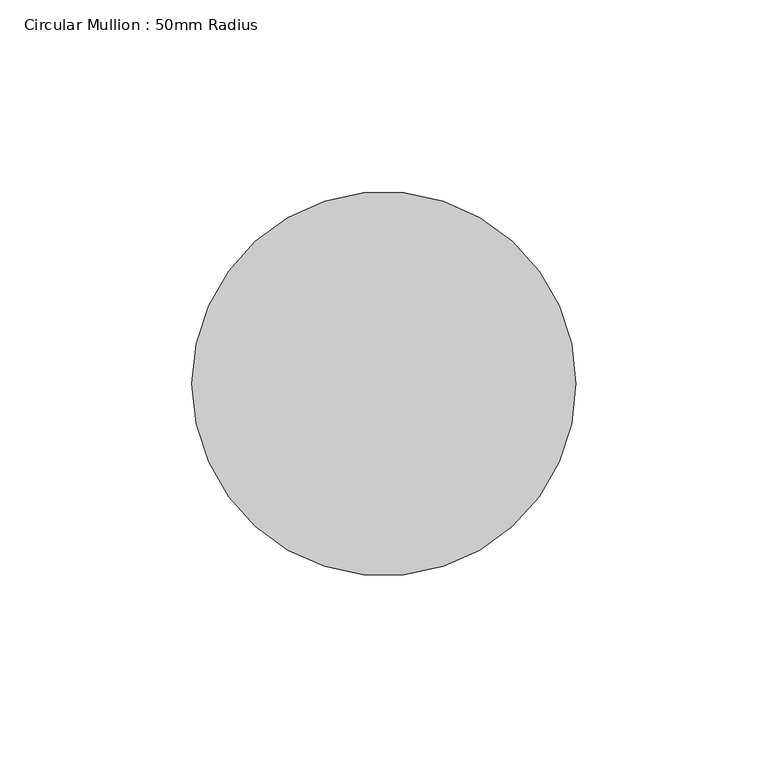
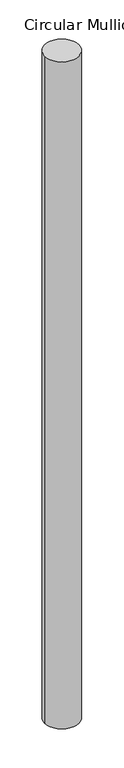
"""IFC4 building model written with IfcOpenShell, lengths in millimetres: member geometry, Circular Mullion : 50mm Radius."""

from ifc_helpers import new_model, si_unit, point, frame, frame_2d, origin, place, context, project, spatial, circle_curve, trimmed, segment, composite_curve, outline, extrude, source, transform, mapped, element, save


def circular_mullion_50mm_radius_993f352e(model_context):
    return source(origin(), model_context, "Body", "SweptSolid", [
        extrude(outline(composite_curve([segment(trimmed(circle_curve(frame_2d((-50.0, 0.0)), 50.0), [point((0.0, 0.0))], [point((-100.0, 0.0))], False, "CARTESIAN"), True, "CONTINUOUS"), segment(trimmed(circle_curve(frame_2d((-50.0, 0.0)), 50.0), [point((-100.0, 0.0))], [point((0.0, 0.0))], False, "CARTESIAN"), True, "CONTINUOUS")], self_intersect=False)), frame((0.0, 0.0, -2050.6614912), z_axis=(0.0, 0.0, 1.0), x_axis=(1.0, 0.0, 0.0)), (0.0, 0.0, 1.0), 2050.6614912),
    ])


if __name__ == "__main__":
    model = new_model("IFC4")
    model_context = context("Model", 3, world=origin())
    ifc_project = project(units=[si_unit("LENGTHUNIT", "METRE", prefix="MILLI")], contexts=[model_context])
    site = spatial("IfcSite", under=ifc_project)
    building = spatial("IfcBuilding", under=site)
    placement = place(None, origin())
    circular_mullion_50mm_radius_shape = circular_mullion_50mm_radius_993f352e(model_context)
    element("IfcMember", 1, ObjectType="Circular Mullion : 50mm Radius", at=placement, inside=building, context=model_context, shape_type="MappedRepresentation", body=[
        mapped(circular_mullion_50mm_radius_shape, transform((0.0, 0.0, 0.0), x_axis=(1.0, 0.0, 0.0), y_axis=(0.0, 1.0, 0.0), z_axis=(0.0, 0.0, 1.0))),
    ])
    save(model, "model.ifc")

# Revit data of these elements
# Type "Circular Mullion : 50mm Radius"
#   built-in parameter 1007350 = 0.164042 (stored number, unit not read)
# Element 1 (IfcMember, "Circular Mullion : 50mm Radius")
#   Materials on its faces: "Aluminium"
# Materials
#   "Aluminium": class "Metal", colour RGB 247 247 247, transparency 0, Description = "Aluminium 6061", Cost = 0
